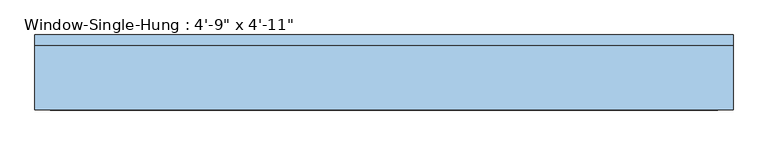
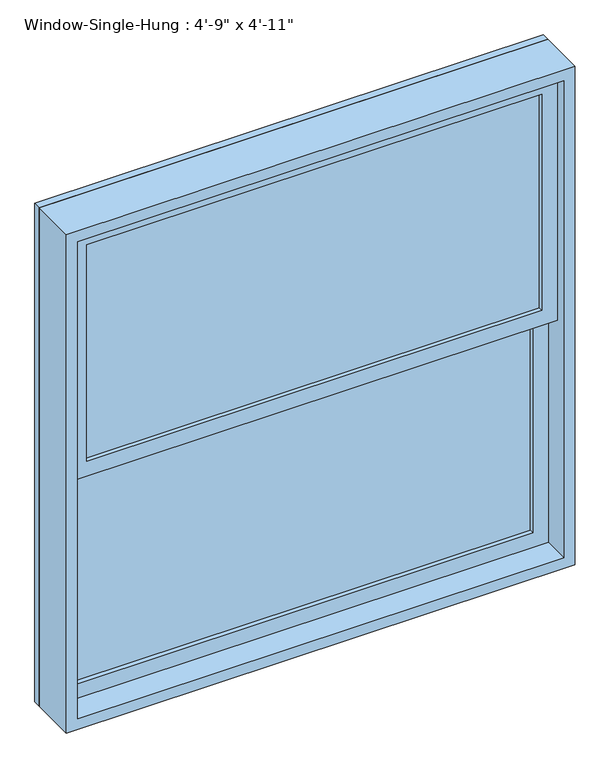
"""IFC4 building model written with IfcOpenShell, lengths in millimetres: window geometry."""

import ifcopenshell
import ifcopenshell.guid

model = None  # the IFC model being written
_history = None  # IfcOwnerHistory: only IFC2X3 demands one
_inside = {}  # id of a spatial element -> (the spatial element, [elements in it])
_under = {}  # id of a project, library or spatial element -> (it, [spatial elements below it])
_declared = {}  # id of a project -> (the project, [libraries it declares])
_typed = {}  # id of a type object -> (the type object, [elements of that type])
_made_of = {}  # id of a material, layer set ... -> (it, [elements and type objects made of it])


def new_model(schema):
    """Start an empty IFC model of exactly this schema.

    Asked for "IFC4X3", IfcOpenShell would pick the latest addendum, in which some entities
    have other attributes; the version numbers below select the first issue.
    IFC2X3 requires an IfcOwnerHistory on every rooted entity: one is made here for all.
    """
    global model, _history
    if schema == "IFC4X3":
        model = ifcopenshell.file(schema_version=(4, 3, 0, 0))
    else:
        model = ifcopenshell.file(schema=schema)
    _inside.clear()
    _under.clear()
    _declared.clear()
    _typed.clear()
    _made_of.clear()
    _history = None
    if model.schema == "IFC2X3":
        org = make("IfcOrganization", Name="unknown")
        user = make(
            "IfcPersonAndOrganization",
            ThePerson=make("IfcPerson", FamilyName="unknown"),
            TheOrganization=org,
        )
        app = make(
            "IfcApplication",
            ApplicationDeveloper=org,
            Version="unknown",
            ApplicationFullName="unknown",
            ApplicationIdentifier="unknown",
        )
        _history = make(
            "IfcOwnerHistory",
            OwningUser=user,
            OwningApplication=app,
            ChangeAction="ADDED",
            CreationDate=0,
        )
    return model


def make(cls, **values):
    """One entity of the class cls with the attributes given. An attribute that is None is left unset."""
    return model.create_entity(
        cls, **{name: value for name, value in values.items() if value is not None}
    )


def rooted(cls, **values):
    """An entity with a GlobalId (a new one), such as an element, a storey or a relation."""
    return make(cls, GlobalId=ifcopenshell.guid.new(), OwnerHistory=_history, **values)


def si_unit(unit_type, name, prefix=None):
    """IfcSIUnit, for example si_unit("LENGTHUNIT", "METRE", prefix="MILLI")."""
    return make("IfcSIUnit", UnitType=unit_type, Prefix=prefix, Name=name)


def assignment(units):
    """IfcUnitAssignment: the units of a project."""
    return None if units is None else make("IfcUnitAssignment", Units=units)


def point(xyz):
    """IfcCartesianPoint."""
    return None if xyz is None else make("IfcCartesianPoint", Coordinates=xyz)


def direction(xyz):
    """IfcDirection."""
    return None if xyz is None else make("IfcDirection", DirectionRatios=xyz)


def frame(location, z_axis=None, x_axis=None):
    """IfcAxis2Placement3D, a coordinate frame: its origin and axes. An axis left out is left unset."""
    return make(
        "IfcAxis2Placement3D",
        Location=point(location),
        Axis=direction(z_axis),
        RefDirection=direction(x_axis),
    )


def origin():
    """The frame at (0, 0, 0) with its axes left unset."""
    return frame((0.0, 0.0, 0.0))


def place(relative_to, where):
    """IfcLocalPlacement: puts the frame where relative to a parent placement (None: the world)."""
    return make(
        "IfcLocalPlacement", PlacementRelTo=relative_to, RelativePlacement=where
    )


def context(
    kind, dimensions, precision=None, world=None, true_north=None, identifier=None
):
    """IfcGeometricRepresentationContext, for example the 3D "Model" context."""
    return make(
        "IfcGeometricRepresentationContext",
        ContextIdentifier=identifier,
        ContextType=kind,
        CoordinateSpaceDimension=dimensions,
        Precision=precision,
        WorldCoordinateSystem=world,
        TrueNorth=true_north,
    )


def project(units=None, contexts=None):
    """IfcProject with its units and contexts."""
    return rooted(
        "IfcProject",
        Name="project",
        RepresentationContexts=contexts,
        UnitsInContext=assignment(units),
    )


def spatial(cls, under=None, at=None, **own):
    """A site, building, storey or space (cls), placed at a placement, below another one or the project."""
    s = rooted(cls, ObjectPlacement=at, **own)
    if under is not None:
        _under.setdefault(under.id(), (under, []))[1].append(s)
    return s


def polyline(points):
    """IfcPolyline through the points."""
    return make("IfcPolyline", Points=[point(p) for p in points])


def outline(outer, holes=None, kind="AREA"):
    """IfcArbitraryClosedProfileDef: a profile drawn as a closed curve; with holes, ...WithVoids."""
    if holes is None:
        return make("IfcArbitraryClosedProfileDef", ProfileType=kind, OuterCurve=outer)
    return make(
        "IfcArbitraryProfileDefWithVoids",
        ProfileType=kind,
        OuterCurve=outer,
        InnerCurves=holes,
    )


def extrude(swept, where, along, depth):
    """IfcExtrudedAreaSolid: the profile swept, set in the frame where, extruded along a direction by depth."""
    return make(
        "IfcExtrudedAreaSolid",
        SweptArea=swept,
        Position=where,
        ExtrudedDirection=direction(along),
        Depth=depth,
    )


def shape(context_of_items, identifier, shape_type, items):
    """IfcShapeRepresentation: the items that make up one representation, for example the "Body"."""
    return make(
        "IfcShapeRepresentation",
        ContextOfItems=context_of_items,
        RepresentationIdentifier=identifier,
        RepresentationType=shape_type,
        Items=items,
    )


def source(mapping_origin, context_of_items, identifier, shape_type, items):
    """IfcRepresentationMap: a shape defined once, which mapped items show again and again."""
    return make(
        "IfcRepresentationMap",
        MappingOrigin=mapping_origin,
        MappedRepresentation=shape(context_of_items, identifier, shape_type, items),
    )


def transform(
    local_origin,
    x_axis=None,
    y_axis=None,
    z_axis=None,
    scale=None,
    scale2=None,
    scale3=None,
    uniform=True,
):
    """IfcCartesianTransformationOperator3D, or its non-uniform kind. x_axis, y_axis, z_axis: its Axis1, 2, 3."""
    if uniform:
        return make(
            "IfcCartesianTransformationOperator3D",
            Axis1=direction(x_axis),
            Axis2=direction(y_axis),
            LocalOrigin=point(local_origin),
            Scale=scale,
            Axis3=direction(z_axis),
        )
    return make(
        "IfcCartesianTransformationOperator3DnonUniform",
        Axis1=direction(x_axis),
        Axis2=direction(y_axis),
        LocalOrigin=point(local_origin),
        Scale=scale,
        Axis3=direction(z_axis),
        Scale2=scale2,
        Scale3=scale3,
    )


def mapped(mapping_source, mapping_target):
    """IfcMappedItem: shows the shape of a source again, moved by a transform."""
    return make(
        "IfcMappedItem", MappingSource=mapping_source, MappingTarget=mapping_target
    )


def made_of(thing, what):
    """Note that an element or type object is made of a material, layer set ...; save() writes the relation."""
    if what is not None:
        _made_of.setdefault(what.id(), (what, []))[1].append(thing)
    return thing


def element(
    cls,
    number,
    at=None,
    inside=None,
    cuts=None,
    type_object=None,
    material=None,
    context=None,
    identifier="Body",
    shape_type=None,
    held_by="IfcProductDefinitionShape",
    body=None,
    shapes=None,
    **own,
):
    """One element of the class cls, such as IfcWall. Its Tag is "e" and its number.

    at: its placement. inside: the storey or other place that contains it. cuts: it is an
    opening in that element (IfcRelVoidsElement). A single representation is given by context,
    identifier, shape_type and body (its items); several are given by shapes. held_by: the class
    of the entity that holds the representations. save() writes the other relations.
    """
    e = rooted(cls, Tag="e%d" % number, ObjectPlacement=at, **own)
    if body is not None:
        shapes = [shape(context, identifier, shape_type, body)]
    if shapes is not None:
        e.Representation = make(held_by, Representations=shapes)
    if inside is not None:
        _inside.setdefault(inside.id(), (inside, []))[1].append(e)
    if cuts is not None:
        rooted(
            "IfcRelVoidsElement", RelatingBuildingElement=cuts, RelatedOpeningElement=e
        )
    if type_object is not None:
        _typed.setdefault(type_object.id(), (type_object, []))[1].append(e)
    return made_of(e, material)


def aggregate(whole, parts):
    """IfcRelAggregates: a whole, such as a stair, and the parts it consists of."""
    return rooted("IfcRelAggregates", RelatingObject=whole, RelatedObjects=parts)


def save(model, path):
    """Write the relations noted so far, then the file.

    IfcRelAggregates (storeys below a building ...), IfcRelContainedInSpatialStructure (elements
    in a storey), IfcRelDefinesByType, IfcRelAssociatesMaterial and IfcRelDeclares: one each for
    every whole, place, type object, material and project.
    """
    for whole, parts in _under.values():
        aggregate(whole, parts)
    for where, things in _inside.values():
        rooted(
            "IfcRelContainedInSpatialStructure",
            RelatedElements=things,
            RelatingStructure=where,
        )
    for kind, things in _typed.values():
        rooted("IfcRelDefinesByType", RelatedObjects=things, RelatingType=kind)
    for what, things in _made_of.values():
        rooted("IfcRelAssociatesMaterial", RelatedObjects=things, RelatingMaterial=what)
    for by, libraries in _declared.values():
        rooted("IfcRelDeclares", RelatingContext=by, RelatedDefinitions=libraries)
    model.write(path)


def window_616431ac(model_context):
    return source(origin(), model_context, "Body", "SweptSolid", [
        extrude(outline(polyline([(647.7, 1.5875), (-647.7, 1.5875), (-647.7, 7.9375), (647.7, 7.9375), (647.7, 1.5875)])), frame((0.0, 0.0, 990.6), z_axis=(0.0, 0.0, 1.0), x_axis=(1.0, 0.0, 0.0)), (0.0, 0.0, 1.0), 650.875),
        extrude(outline(polyline([(-647.7, 14.2875), (-647.7, 20.6375), (647.7, 20.6375), (647.7, 14.2875), (-647.7, 14.2875)])), frame((0.0, 0.0, 990.6), z_axis=(0.0, 0.0, 1.0), x_axis=(1.0, 0.0, 0.0)), (0.0, 0.0, 1.0), 650.875),
        extrude(outline(polyline([(647.7, -42.8625), (-647.7, -42.8625), (-647.7, -36.5125), (647.7, -36.5125), (647.7, -42.8625)])), frame((0.0, 0.0, 1685.925), z_axis=(0.0, 0.0, 1.0), x_axis=(1.0, 0.0, 0.0)), (0.0, 0.0, 1.0), 650.875),
        extrude(outline(polyline([(-647.7, -30.1625), (-647.7, -23.8125), (647.7, -23.8125), (647.7, -30.1625), (-647.7, -30.1625)])), frame((0.0, 0.0, 1685.925), z_axis=(0.0, 0.0, 1.0), x_axis=(1.0, 0.0, 0.0)), (0.0, 0.0, 1.0), 650.875),
        extrude(outline(polyline([(1685.925, 692.15), (1685.925, -692.15), (946.15, -692.15), (946.15, 692.15), (1685.925, 692.15)]), holes=[polyline([(1641.475, -647.7), (1641.475, 647.7), (990.6, 647.7), (990.6, -647.7), (1641.475, -647.7)])]), frame((0.0, -11.1125, 0.0), z_axis=(0.0, 1.0, 0.0), x_axis=(0.0, 0.0, 1.0)), (0.0, 0.0, 1.0), 44.45),
        extrude(outline(polyline([(2381.25, 692.15), (2381.25, -692.15), (1641.475, -692.15), (1641.475, 692.15), (2381.25, 692.15)]), holes=[polyline([(2336.8, -647.7), (2336.8, 647.7), (1685.925, 647.7), (1685.925, -647.7), (2336.8, -647.7)])]), frame((0.0, -55.5625, 0.0), z_axis=(0.0, 1.0, 0.0), x_axis=(0.0, 0.0, 1.0)), (0.0, 0.0, 1.0), 44.45),
        extrude(outline(polyline([(2413.0, 723.9), (2413.0, -723.9), (914.4, -723.9), (914.4, 723.9), (2413.0, 723.9)]), holes=[polyline([(2381.25, -692.15), (2381.25, 692.15), (946.15, 692.15), (946.15, -692.15), (2381.25, -692.15)])]), frame((0.0, -87.3125, 0.0), z_axis=(0.0, 1.0, 0.0), x_axis=(0.0, 0.0, 1.0)), (0.0, 0.0, 1.0), 133.35),
        extrude(outline(polyline([(2413.0, 723.9), (2413.0, -723.9), (914.4, -723.9), (914.4, 723.9), (2413.0, 723.9)]), holes=[polyline([(2393.95, 704.85), (933.45, 704.85), (933.45, -704.85), (2393.95, -704.85), (2393.95, 704.85)])]), frame((0.0, 46.0375, 0.0), z_axis=(0.0, 1.0, 0.0), x_axis=(0.0, 0.0, 1.0)), (0.0, 0.0, 1.0), 22.225),
    ])


if __name__ == "__main__":
    model = new_model("IFC4")
    model_context = context("Model", 3, world=origin())
    ifc_project = project(units=[si_unit("LENGTHUNIT", "METRE", prefix="MILLI")], contexts=[model_context])
    site = spatial("IfcSite", under=ifc_project)
    building = spatial("IfcBuilding", under=site)
    placement = place(None, origin())
    window_shape = window_616431ac(model_context)
    element("IfcWindow", 1, ObjectType="Window-Single-Hung : 4'-9\" x 4'-11\"", at=placement, inside=building, context=model_context, shape_type="MappedRepresentation", body=[
        mapped(window_shape, transform((0.0, 0.0, 0.0), x_axis=(1.0, 0.0, 0.0), y_axis=(0.0, 1.0, 0.0), z_axis=(0.0, 0.0, 1.0))),
    ])
    save(model, "model.ifc")

# Revit data of these elements
# Type "Window-Single-Hung : 4'-9\" x 4'-11\""
#   Type Mark = "23"
#   Fire Rating = "0.5h"
#   Construction Type Id = "DG-DR"
#   Assembly Code = "B2020100"
#   Analytic Construction = "Double glazing - domestic"
#   Wall Thickness [instance default] = 0' - 6"
#   Window Inset [instance default] = 0' - 0"
#   Visual Light Transmittance = 0.81
#   Thermal Resistance (R) = 0.319569 (m²·K)/W
#   Solar Heat Gain Coefficient = 0.76
#   Muntin Width = 4' - 3"
#   Muntin Height = 2' - 1 5/8"
#   Interior Wall Closure [instance default] = 0' - 1 1/2"
#   Rough Width = 4' - 9 1/2"
#   Rough Height = 4' - 11 1/2"
#   Frame Extension [instance default] = 0' - 1 1/4"
#   Exterior Wall Closure [instance default] = 0' - 0 1/2"
#   Extension Jamb [instance default] = 0' - 1 1/2"
#   Heat Transfer Coefficient (U) = 3.12929 W/(m²·K)
#   Height = 4' - 11"
#   Width = 4' - 9"
#   Top Muntin Visibility = yes
#   Indicator Visibility [instance default] = yes
#   Extension Jamb Visibility [instance default] = yes
#   Interior Trim Visibility [instance default] = yes
#   Exterior Trim Visibility [instance default] = yes
#   Bottom Muntin Visibility = yes
#   Muntin Pattern = Muntin Pattern_2x2 : Muntin Pattern_2x2
#   Interior Trim Material = Wood - Stained
#   Interior Trim = Trim-Window-Interior-Flat : Picture Frame
#   Exterior Trim Material = Clad - White
#   Exterior Trim = Trim-Window-Exterior-Flat : with Sill
#   Glass Panel Material = Glass
#   Exterior Frame Material = Clad - White
#   Interior Frame Material = Wood - Stained
#   Wall Closure = (empty or 0)
# Element 1 (IfcWindow, "Window-Single-Hung : 4'-9\" x 4'-11\"")
#   Wall Thickness = 0' - 5 3/8"
#   Extension Jamb = 0' - 0 7/8"
#   Materials on its faces: "Wood - Stained", "Glass", "Clad - White"
# Materials
#   "Wood - Stained": class "Wood", colour RGB 224 178 126, transparency 0, Cost = 0
#   "Clad - White": class "Wood", colour RGB 242 242 238, transparency 0, Cost = 0
#   "Glass": class "Glass", colour RGB 0 128 192, transparency 0.75, Description = "Soda Lime Glass", Cost = 0
